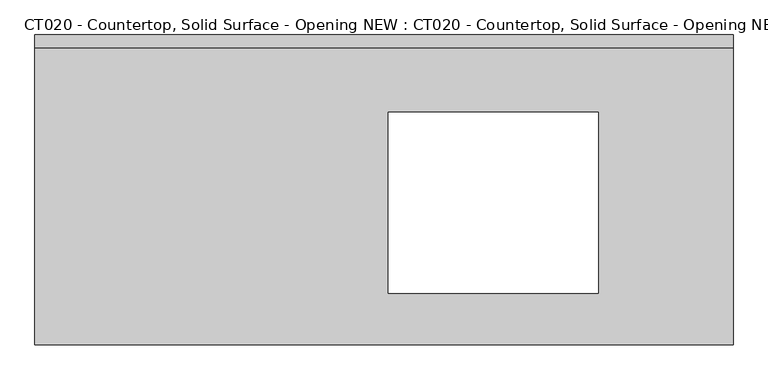
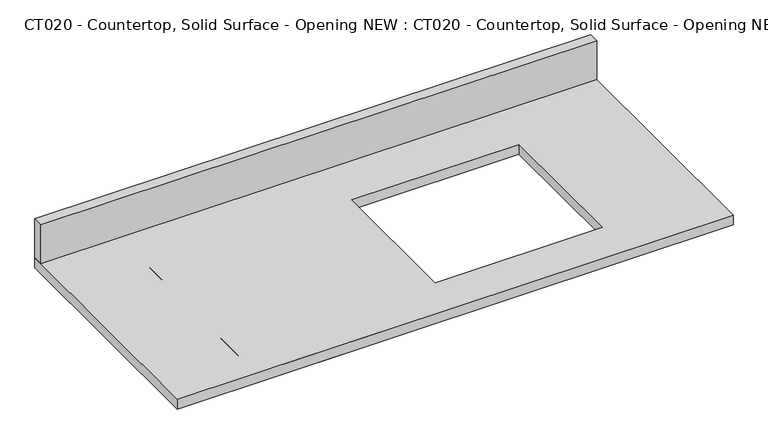
"""IFC4 building model written with IfcOpenShell, lengths in millimetres: proxy geometry, CT020 - Countertop, Solid Surface - Opening NEW : CT020 - Countertop, Solid Surface - Opening NEW."""

from ifc_helpers import new_model, si_unit, frame, origin, origin_with_axes, place, context, project, spatial, polyline, outline, extrude, source, transform, mapped, element, save


def ct020_countertop_solid_surface_opening_new_ct020_countertop_6df85a66(model_context):
    return source(origin(), model_context, "Body", "SweptSolid", [
        extrude(outline(polyline([(1027.3092306, 304.8), (1027.3092306, -304.8), (-346.4474741, -304.8), (-346.4474741, 304.8), (1027.3092306, 304.8)]), holes=[polyline([(762.0, 152.9546125), (349.25, 152.9546125), (349.25, -203.2), (762.0, -203.2), (762.0, 152.9546125)])]), origin_with_axes(), (0.0, 0.0, 1.0), 25.4),
        extrude(outline(polyline([(-346.4474741, 279.4), (-346.4474741, 304.8), (1027.3092306, 304.8), (1027.3092306, 279.4), (-346.4474741, 279.4)])), frame((0.0, 0.0, 25.4), z_axis=(0.0, 0.0, 1.0), x_axis=(1.0, 0.0, 0.0)), (0.0, 0.0, 1.0), 101.6),
        extrude(outline(polyline([(-152.4, 304.8), (152.4, 304.8), (152.4, -304.8), (-152.4, -304.8), (-152.4, 0.0), (-152.4, 304.8)])), origin_with_axes(), (0.0, 0.0, 1.0), 25.4),
    ])


if __name__ == "__main__":
    model = new_model("IFC4")
    model_context = context("Model", 3, world=origin())
    ifc_project = project(units=[si_unit("LENGTHUNIT", "METRE", prefix="MILLI")], contexts=[model_context])
    site = spatial("IfcSite", under=ifc_project)
    building = spatial("IfcBuilding", under=site)
    placement = place(None, origin())
    ct020_countertop_solid_surface_opening_new_ct020_countertop_shape = ct020_countertop_solid_surface_opening_new_ct020_countertop_6df85a66(model_context)
    element("IfcBuildingElementProxy", 1, Name="CT020 - Countertop, Solid Surface - Opening NEW : CT020 - Countertop, Solid Surface - Opening NEW", ObjectType="CT020 - Countertop, Solid Surface - Opening NEW : CT020 - Countertop, Solid Surface - Opening NEW", at=placement, inside=building, context=model_context, shape_type="MappedRepresentation", body=[
        mapped(ct020_countertop_solid_surface_opening_new_ct020_countertop_shape, transform((0.0, 0.0, 0.0), x_axis=(1.0, 0.0, 0.0), y_axis=(0.0, 1.0, 0.0), z_axis=(0.0, 0.0, 1.0))),
    ])
    save(model, "model.ifc")

# Revit data of these elements
# Type "CT020 - Countertop, Solid Surface - Opening NEW : CT020 - Countertop, Solid Surface - Opening NEW"
#   Watts2 = "0"
#   Watts1 = "0"
#   Unit_Issue = "LF"
#   UTIL_6_Misc = "-"
#   UTIL_5_NonMedGas = "-"
#   UTIL_4_MiscGas = "-"
#   UTIL_3_MedGas = "-"
#   UTIL_2_Elec = "-"
#   UTIL_1_WaterDrain = "-"
#   Nomenclature = "Countertop, Solid Surface"
#   NSN = "6530"
#   Location [instance default] = ""
#   JSN = "CT020"
#   Fund_Source_VA = "-"
#   Fund_Source_Navy = "-"
#   Fund_Source_Army = "-"
#   Fund_Source_AF = "-"
#   ELEC_Volts2 = "0"
#   ELEC_Volts1 = "0"
#   ELEC_Phase2 = "0"
#   ELEC_Phase1 = "0"
#   ELEC_HertzSwitch = "0"
#   ELEC_HertzDependent = "0"
#   ELEC_Hertz = "0"
#   ELEC_Amps2 = "0"
#   ELEC_Amps1 = "0"
#   DetailDescription = "High pressure laminate countertop (composition of wood particle core with plastic laminate surface) having a hard smooth surface finish, standard thickness of 1\", and a 4\" butt backsplash/curb. Also referred to as a work surface or work top. Available in a wide choice of colors, patterns, and depths. Used in general purpose areas requiring a basic work surface arrangement with limited heat resistance and poor chemical resistance. Pricing based upon a 24\" depth."
#   CAT_VA = "A"
#   CAT_Navy = "A"
#   CAT_IHS = "-"
#   CAT_Army = "A"
#   CAT_AF = "A"
#   BTUperhour = "0"
#   Weight_IP = 14
#   OpeningLength2 [instance default] = 1' - 6"
#   OpeningLength [instance default] = 3' - 2"
#   OpeningDepth2 [instance default] = 0' - 8"
#   OpeningDepth [instance default] = 0' - 8"
#   DIM_Width_IP = 1' - 0"
#   DIM_Height_IP = 0' - 1"
#   DIM_Depth_IP = 2' - 0"
#   CustomLength2 [instance default] = 3' - 0"
#   CustomLength [instance default] = 3' - 0"
#   Assembly Code = ""
# Element 1 (IfcBuildingElementProxy, "CT020 - Countertop, Solid Surface - Opening NEW : CT020 - Countertop, Solid Surface - Opening NEW")
#   OpeningLength2 = 0' - 4 1/4"
#   OpeningLength = 1' - 0"
#   OpeningDepth2 = 0' - 6.02184"
#   CustomLength2 = 3' - 4.44525"
#   CustomLength = 1' - 1.63966"
#   Materials on its faces: "CounterTopFinish", "EquipSpace"
# Materials
#   "CounterTopFinish": class "Unassigned", colour RGB 139 121 96, transparency 0
#   "EquipSpace": class "Unassigned", colour RGB 221 217 195, transparency 0.5
